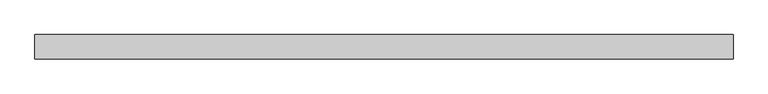
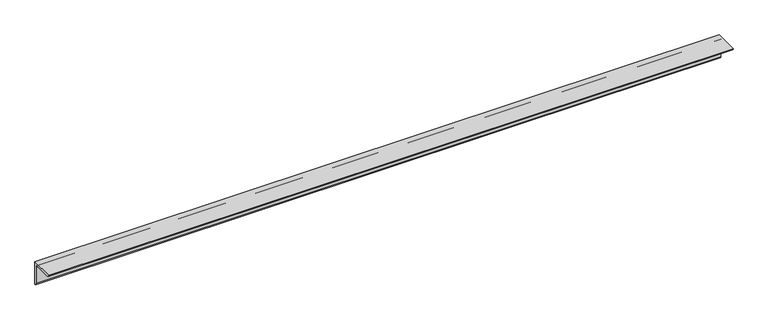
"""IFC4 building model written with IfcOpenShell, lengths in millimetres: member geometry, 0912_Steel Framing_L-KSD3502 : H_SB_AR_S03_L-130x130x12_HBR3."""

import ifcopenshell
import ifcopenshell.guid

model = None  # the IFC model being written
_history = None  # IfcOwnerHistory: only IFC2X3 demands one
_inside = {}  # id of a spatial element -> (the spatial element, [elements in it])
_under = {}  # id of a project, library or spatial element -> (it, [spatial elements below it])
_declared = {}  # id of a project -> (the project, [libraries it declares])
_typed = {}  # id of a type object -> (the type object, [elements of that type])
_made_of = {}  # id of a material, layer set ... -> (it, [elements and type objects made of it])


def new_model(schema):
    """Start an empty IFC model of exactly this schema.

    Asked for "IFC4X3", IfcOpenShell would pick the latest addendum, in which some entities
    have other attributes; the version numbers below select the first issue.
    IFC2X3 requires an IfcOwnerHistory on every rooted entity: one is made here for all.
    """
    global model, _history
    if schema == "IFC4X3":
        model = ifcopenshell.file(schema_version=(4, 3, 0, 0))
    else:
        model = ifcopenshell.file(schema=schema)
    _inside.clear()
    _under.clear()
    _declared.clear()
    _typed.clear()
    _made_of.clear()
    _history = None
    if model.schema == "IFC2X3":
        org = make("IfcOrganization", Name="unknown")
        user = make(
            "IfcPersonAndOrganization",
            ThePerson=make("IfcPerson", FamilyName="unknown"),
            TheOrganization=org,
        )
        app = make(
            "IfcApplication",
            ApplicationDeveloper=org,
            Version="unknown",
            ApplicationFullName="unknown",
            ApplicationIdentifier="unknown",
        )
        _history = make(
            "IfcOwnerHistory",
            OwningUser=user,
            OwningApplication=app,
            ChangeAction="ADDED",
            CreationDate=0,
        )
    return model


def make(cls, **values):
    """One entity of the class cls with the attributes given. An attribute that is None is left unset."""
    return model.create_entity(
        cls, **{name: value for name, value in values.items() if value is not None}
    )


def rooted(cls, **values):
    """An entity with a GlobalId (a new one), such as an element, a storey or a relation."""
    return make(cls, GlobalId=ifcopenshell.guid.new(), OwnerHistory=_history, **values)


def si_unit(unit_type, name, prefix=None):
    """IfcSIUnit, for example si_unit("LENGTHUNIT", "METRE", prefix="MILLI")."""
    return make("IfcSIUnit", UnitType=unit_type, Prefix=prefix, Name=name)


def assignment(units):
    """IfcUnitAssignment: the units of a project."""
    return None if units is None else make("IfcUnitAssignment", Units=units)


def point(xyz):
    """IfcCartesianPoint."""
    return None if xyz is None else make("IfcCartesianPoint", Coordinates=xyz)


def direction(xyz):
    """IfcDirection."""
    return None if xyz is None else make("IfcDirection", DirectionRatios=xyz)


def frame(location, z_axis=None, x_axis=None):
    """IfcAxis2Placement3D, a coordinate frame: its origin and axes. An axis left out is left unset."""
    return make(
        "IfcAxis2Placement3D",
        Location=point(location),
        Axis=direction(z_axis),
        RefDirection=direction(x_axis),
    )


def frame_2d(location, x_axis=None):
    """IfcAxis2Placement2D, a coordinate frame in the plane: its origin and x axis."""
    return make(
        "IfcAxis2Placement2D", Location=point(location), RefDirection=direction(x_axis)
    )


def origin():
    """The frame at (0, 0, 0) with its axes left unset."""
    return frame((0.0, 0.0, 0.0))


def place(relative_to, where):
    """IfcLocalPlacement: puts the frame where relative to a parent placement (None: the world)."""
    return make(
        "IfcLocalPlacement", PlacementRelTo=relative_to, RelativePlacement=where
    )


def context(
    kind, dimensions, precision=None, world=None, true_north=None, identifier=None
):
    """IfcGeometricRepresentationContext, for example the 3D "Model" context."""
    return make(
        "IfcGeometricRepresentationContext",
        ContextIdentifier=identifier,
        ContextType=kind,
        CoordinateSpaceDimension=dimensions,
        Precision=precision,
        WorldCoordinateSystem=world,
        TrueNorth=true_north,
    )


def project(units=None, contexts=None):
    """IfcProject with its units and contexts."""
    return rooted(
        "IfcProject",
        Name="project",
        RepresentationContexts=contexts,
        UnitsInContext=assignment(units),
    )


def spatial(cls, under=None, at=None, **own):
    """A site, building, storey or space (cls), placed at a placement, below another one or the project."""
    s = rooted(cls, ObjectPlacement=at, **own)
    if under is not None:
        _under.setdefault(under.id(), (under, []))[1].append(s)
    return s


def polyline(points):
    """IfcPolyline through the points."""
    return make("IfcPolyline", Points=[point(p) for p in points])


def circle_curve(where, radius):
    """IfcCircle in the frame where."""
    return make("IfcCircle", Position=where, Radius=radius)


def trimmed(basis, trim1, trim2, sense, master):
    """IfcTrimmedCurve: the piece of a basis curve between two trims."""
    return make(
        "IfcTrimmedCurve",
        BasisCurve=basis,
        Trim1=trim1,
        Trim2=trim2,
        SenseAgreement=sense,
        MasterRepresentation=master,
    )


def segment(curve, same_sense, transition):
    """IfcCompositeCurveSegment."""
    return make(
        "IfcCompositeCurveSegment",
        Transition=transition,
        SameSense=same_sense,
        ParentCurve=curve,
    )


def composite_curve(segments, self_intersect=None):
    """IfcCompositeCurve: segments joined end to end."""
    return make("IfcCompositeCurve", Segments=segments, SelfIntersect=self_intersect)


def outline(outer, holes=None, kind="AREA"):
    """IfcArbitraryClosedProfileDef: a profile drawn as a closed curve; with holes, ...WithVoids."""
    if holes is None:
        return make("IfcArbitraryClosedProfileDef", ProfileType=kind, OuterCurve=outer)
    return make(
        "IfcArbitraryProfileDefWithVoids",
        ProfileType=kind,
        OuterCurve=outer,
        InnerCurves=holes,
    )


def extrude(swept, where, along, depth):
    """IfcExtrudedAreaSolid: the profile swept, set in the frame where, extruded along a direction by depth."""
    return make(
        "IfcExtrudedAreaSolid",
        SweptArea=swept,
        Position=where,
        ExtrudedDirection=direction(along),
        Depth=depth,
    )


def shape(context_of_items, identifier, shape_type, items):
    """IfcShapeRepresentation: the items that make up one representation, for example the "Body"."""
    return make(
        "IfcShapeRepresentation",
        ContextOfItems=context_of_items,
        RepresentationIdentifier=identifier,
        RepresentationType=shape_type,
        Items=items,
    )


def source(mapping_origin, context_of_items, identifier, shape_type, items):
    """IfcRepresentationMap: a shape defined once, which mapped items show again and again."""
    return make(
        "IfcRepresentationMap",
        MappingOrigin=mapping_origin,
        MappedRepresentation=shape(context_of_items, identifier, shape_type, items),
    )


def transform(
    local_origin,
    x_axis=None,
    y_axis=None,
    z_axis=None,
    scale=None,
    scale2=None,
    scale3=None,
    uniform=True,
):
    """IfcCartesianTransformationOperator3D, or its non-uniform kind. x_axis, y_axis, z_axis: its Axis1, 2, 3."""
    if uniform:
        return make(
            "IfcCartesianTransformationOperator3D",
            Axis1=direction(x_axis),
            Axis2=direction(y_axis),
            LocalOrigin=point(local_origin),
            Scale=scale,
            Axis3=direction(z_axis),
        )
    return make(
        "IfcCartesianTransformationOperator3DnonUniform",
        Axis1=direction(x_axis),
        Axis2=direction(y_axis),
        LocalOrigin=point(local_origin),
        Scale=scale,
        Axis3=direction(z_axis),
        Scale2=scale2,
        Scale3=scale3,
    )


def mapped(mapping_source, mapping_target):
    """IfcMappedItem: shows the shape of a source again, moved by a transform."""
    return make(
        "IfcMappedItem", MappingSource=mapping_source, MappingTarget=mapping_target
    )


def made_of(thing, what):
    """Note that an element or type object is made of a material, layer set ...; save() writes the relation."""
    if what is not None:
        _made_of.setdefault(what.id(), (what, []))[1].append(thing)
    return thing


def element(
    cls,
    number,
    at=None,
    inside=None,
    cuts=None,
    type_object=None,
    material=None,
    context=None,
    identifier="Body",
    shape_type=None,
    held_by="IfcProductDefinitionShape",
    body=None,
    shapes=None,
    **own,
):
    """One element of the class cls, such as IfcWall. Its Tag is "e" and its number.

    at: its placement. inside: the storey or other place that contains it. cuts: it is an
    opening in that element (IfcRelVoidsElement). A single representation is given by context,
    identifier, shape_type and body (its items); several are given by shapes. held_by: the class
    of the entity that holds the representations. save() writes the other relations.
    """
    e = rooted(cls, Tag="e%d" % number, ObjectPlacement=at, **own)
    if body is not None:
        shapes = [shape(context, identifier, shape_type, body)]
    if shapes is not None:
        e.Representation = make(held_by, Representations=shapes)
    if inside is not None:
        _inside.setdefault(inside.id(), (inside, []))[1].append(e)
    if cuts is not None:
        rooted(
            "IfcRelVoidsElement", RelatingBuildingElement=cuts, RelatedOpeningElement=e
        )
    if type_object is not None:
        _typed.setdefault(type_object.id(), (type_object, []))[1].append(e)
    return made_of(e, material)


def aggregate(whole, parts):
    """IfcRelAggregates: a whole, such as a stair, and the parts it consists of."""
    return rooted("IfcRelAggregates", RelatingObject=whole, RelatedObjects=parts)


def save(model, path):
    """Write the relations noted so far, then the file.

    IfcRelAggregates (storeys below a building ...), IfcRelContainedInSpatialStructure (elements
    in a storey), IfcRelDefinesByType, IfcRelAssociatesMaterial and IfcRelDeclares: one each for
    every whole, place, type object, material and project.
    """
    for whole, parts in _under.values():
        aggregate(whole, parts)
    for where, things in _inside.values():
        rooted(
            "IfcRelContainedInSpatialStructure",
            RelatedElements=things,
            RelatingStructure=where,
        )
    for kind, things in _typed.values():
        rooted("IfcRelDefinesByType", RelatedObjects=things, RelatingType=kind)
    for what, things in _made_of.values():
        rooted("IfcRelAssociatesMaterial", RelatedObjects=things, RelatingMaterial=what)
    for by, libraries in _declared.values():
        rooted("IfcRelDeclares", RelatingContext=by, RelatedDefinitions=libraries)
    model.write(path)


def member_c049ea03(model_context):
    return source(origin(), model_context, "Body", "SweptSolid", [
        extrude(outline(composite_curve([segment(polyline([(36.4, 36.4), (36.4, -93.6)]), True, "CONTINUOUS"), segment(trimmed(circle_curve(frame_2d((36.4, -81.6)), 12.0), [point((36.4, -93.6))], [point((24.4, -81.6))], False, "CARTESIAN"), True, "CONTINUOUS"), segment(polyline([(24.4, -81.6), (24.4, 12.4)]), True, "CONTINUOUS"), segment(trimmed(circle_curve(frame_2d((12.4, 12.4)), 12.0), [point((24.4, 12.4))], [point((12.4, 24.4))], True, "CARTESIAN"), True, "CONTINUOUS"), segment(polyline([(12.4, 24.4), (-81.6, 24.4)]), True, "CONTINUOUS"), segment(trimmed(circle_curve(frame_2d((-81.6, 36.4)), 12.0), [point((-81.6, 24.4))], [point((-93.6, 36.4))], False, "CARTESIAN"), True, "CONTINUOUS"), segment(polyline([(-93.6, 36.4), (36.4, 36.4)]), True, "CONTINUOUS")], self_intersect=False)), frame((-1867.6865023, 0.0, 0.0), z_axis=(1.0, 0.0, 0.0), x_axis=(0.0, 1.0, 0.0)), (0.0, 0.0, 1.0), 3720.541926),
    ])


if __name__ == "__main__":
    model = new_model("IFC4")
    model_context = context("Model", 3, world=origin())
    ifc_project = project(units=[si_unit("LENGTHUNIT", "METRE", prefix="MILLI")], contexts=[model_context])
    site = spatial("IfcSite", under=ifc_project)
    building = spatial("IfcBuilding", under=site)
    placement = place(None, origin())
    member_shape = member_c049ea03(model_context)
    element("IfcMember", 1, ObjectType="0912_Steel Framing_L-KSD3502 : H_SB_AR_S03_L-130x130x12_HBR3", at=placement, inside=building, context=model_context, shape_type="MappedRepresentation", body=[
        mapped(member_shape, transform((0.0, 0.0, 0.0), x_axis=(1.0, 0.0, 0.0), y_axis=(0.0, 1.0, 0.0), z_axis=(0.0, 0.0, 1.0))),
    ])
    save(model, "model.ifc")

# Revit data of these elements
# Type "0912_Steel Framing_L-KSD3502 : H_SB_AR_S03_L-130x130x12_HBR3"
#   k = 25 mm
#   Perimeter = 0.52 m²/m
#   Nominal Weight = 23.40 kgf/m
#   Length [instance default] = 1000 mm
#   b = 130 mm
#   d = 130 mm
#   t = 12 mm
#   x = 36.4 mm
#   y = 36.4 mm
#   A = 2976.00 m²
#   Structural Material [instance default] = Steel, 45-345
# Element 1 (IfcMember, "0912_Steel Framing_L-KSD3502 : H_SB_AR_S03_L-130x130x12_HBR3")
#   Structural Material = Steel ASTM A36
#   Materials on its faces: "Steel ASTM A36"
# Materials
#   "Steel, 45-345": class "Metal", colour RGB 189 187 185, transparency 0, Description = "Steel 345 MPa", Cost = 0
#   "Steel ASTM A36": class "Metal", colour RGB 199 199 199, transparency 0, Description = "Structural steel, ASTM A36 Grade B, mill finish", Cost = 0
